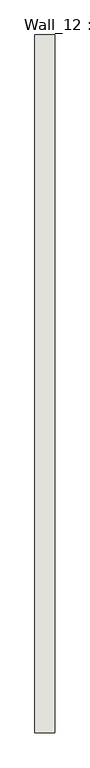
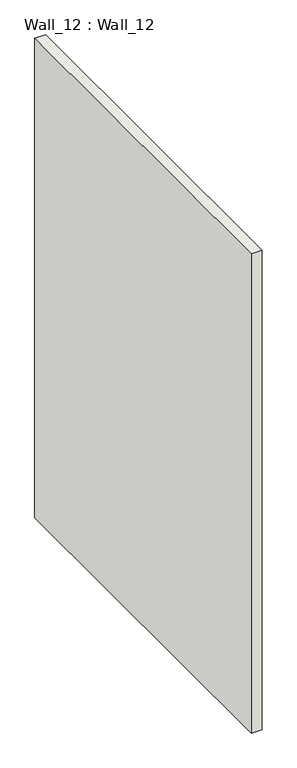
"""IFC4 building model written with IfcOpenShell, lengths in millimetres: wall geometry, Wall_12 : Wall_12."""

from ifc_helpers import new_model, si_unit, origin, origin_with_axes, place, context, project, spatial, polyline, outline, extrude, source, transform, mapped, element, save


def wall_12_wall_12_6134a25a(model_context):
    return source(origin(), model_context, "Body", "SweptSolid", [
        extrude(outline(polyline([(4900.0, 7630.0), (4900.0, 4150.0), (4800.0, 4150.0), (4800.0, 7630.0), (4900.0, 7630.0)])), origin_with_axes(), (0.0, 0.0, 1.0), 4700.0),
    ])


if __name__ == "__main__":
    model = new_model("IFC4")
    model_context = context("Model", 3, world=origin())
    ifc_project = project(units=[si_unit("LENGTHUNIT", "METRE", prefix="MILLI")], contexts=[model_context])
    site = spatial("IfcSite", under=ifc_project)
    building = spatial("IfcBuilding", under=site)
    placement = place(None, origin())
    wall_12_wall_12_shape = wall_12_wall_12_6134a25a(model_context)
    element("IfcWall", 1, ObjectType="Wall_12 : Wall_12", at=placement, inside=building, context=model_context, shape_type="MappedRepresentation", body=[
        mapped(wall_12_wall_12_shape, transform((0.0, 0.0, 0.0), x_axis=(1.0, 0.0, 0.0), y_axis=(0.0, 1.0, 0.0), z_axis=(0.0, 0.0, 1.0))),
    ])
    save(model, "model.ifc")

# Revit data of these elements
# Type "Wall_12 : Wall_12"
#   NameOverride = "Wall_12"
# Element 1 (IfcWall, "Wall_12 : Wall_12")
#   Materials on its faces: "IfcSurfaceStyle #33"
# Materials
#   "IfcSurfaceStyle #33": class "Unassigned", colour RGB 214 214 214, transparency 0
